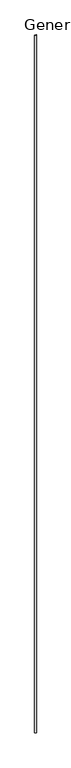
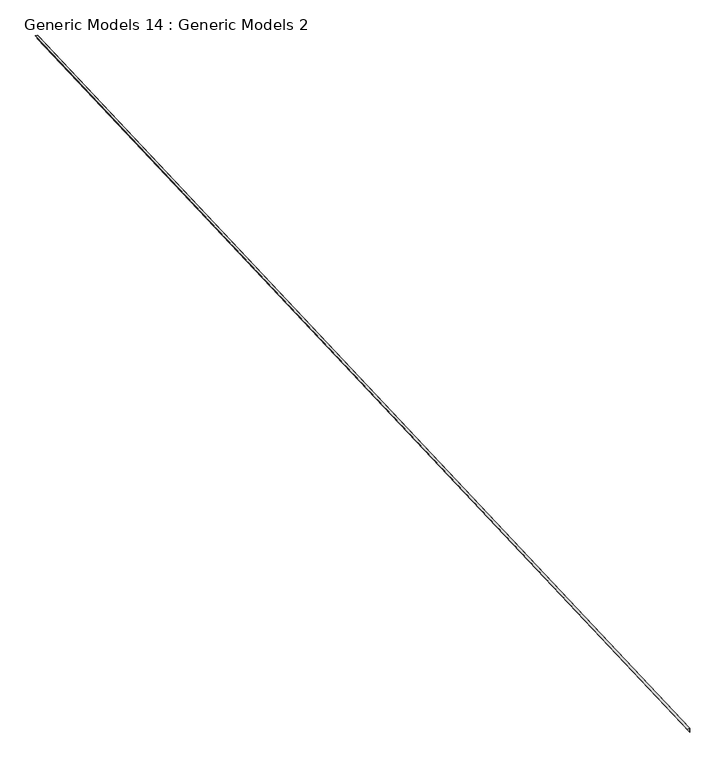
"""IFC4 building model written with IfcOpenShell, lengths in millimetres: proxy geometry, Generic Models 14 : Generic Models 2."""

from ifc_helpers import new_model, si_unit, frame, origin, place, context, project, spatial, polyline, outline, extrude, source, transform, mapped, element, save


def generic_models_14_generic_models_2_2a3970c4(model_context):
    return source(origin(), model_context, "Body", "SweptSolid", [
        extrude(outline(polyline([(-124.2117854, 0.0), (0.0, 0.0), (0.0, -1.5875), (-125.7992854, -1.5875), (-125.7992854, 74.7707967), (-124.2117854, 74.7707967), (-124.2117854, 0.0)])), frame((667547.3117239, -569969.9605331, 8562.7994962), z_axis=(0.0, 0.9991330730923521, 0.041630544712176844), x_axis=(0.0, 0.041630544712176844, -0.9991330730923521)), (0.0, 0.0, 1.0), 33406.7702703),
    ])


if __name__ == "__main__":
    model = new_model("IFC4")
    model_context = context("Model", 3, world=origin())
    ifc_project = project(units=[si_unit("LENGTHUNIT", "METRE", prefix="MILLI")], contexts=[model_context])
    site = spatial("IfcSite", under=ifc_project)
    building = spatial("IfcBuilding", under=site)
    placement = place(None, origin())
    generic_models_14_generic_models_2_shape = generic_models_14_generic_models_2_2a3970c4(model_context)
    element("IfcBuildingElementProxy", 1, Name="Generic Models 14 : Generic Models 2", ObjectType="Generic Models 14 : Generic Models 2", at=placement, inside=building, context=model_context, shape_type="MappedRepresentation", body=[
        mapped(generic_models_14_generic_models_2_shape, transform((0.0, 0.0, 0.0), x_axis=(1.0, 0.0, 0.0), y_axis=(0.0, 1.0, 0.0), z_axis=(0.0, 0.0, 1.0))),
    ])
    save(model, "model.ifc")

# Revit data of these elements
# Element 1 (IfcBuildingElementProxy, "Generic Models 14 : Generic Models 2")
#   Materials on its faces: "RAKE ANGLE - SEE STRUCT. DWGs"
# Materials
#   "RAKE ANGLE - SEE STRUCT. DWGs": class "Unassigned", colour RGB 210 209 208, transparency 0, Cost = 0
